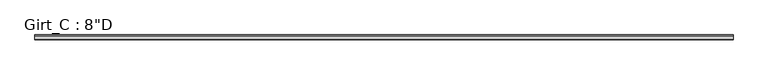
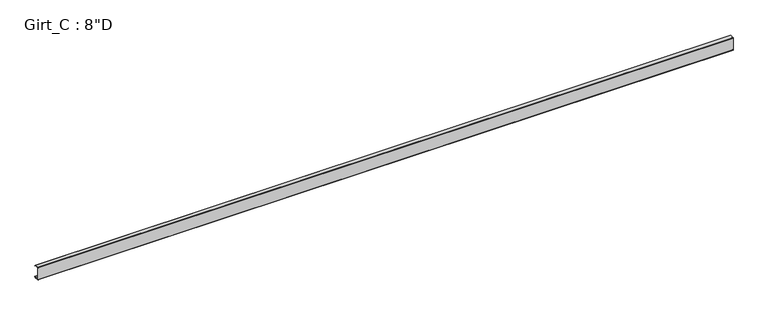
"""IFC4 building model written with IfcOpenShell, lengths in millimetres: beam geometry."""

from ifc_helpers import new_model, si_unit, point, frame, frame_2d, origin, place, context, project, spatial, polyline, circle_curve, trimmed, segment, composite_curve, outline, extrude, source, transform, mapped, element, save


def beam_d1ffb292(model_context):
    return source(origin(), model_context, "Body", "SweptSolid", [
        extrude(outline(composite_curve([segment(polyline([(63.5, 101.6), (75.745104, 87.0068534), (73.6169367, 85.221109), (62.204539, 98.821875), (3.3005807, 98.821875)]), True, "CONTINUOUS"), segment(trimmed(circle_curve(frame_2d((3.3741066, 96.8381931)), 1.9850441), [point((3.3005807, 98.821875))], [point((1.3890625, 96.8381931))], True, "CARTESIAN"), True, "CONTINUOUS"), segment(polyline([(1.3890625, 96.8381931), (1.3890625, -96.8389339)]), True, "CONTINUOUS"), segment(trimmed(circle_curve(frame_2d((3.3748024, -96.8389339)), 1.9857399), [point((1.3890625, -96.8389339))], [point((3.2694106, -98.821875))], True, "CARTESIAN"), True, "CONTINUOUS"), segment(polyline([(3.2694106, -98.821875), (62.204539, -98.821875), (73.6169367, -85.221109), (75.745104, -87.0068534), (63.5, -101.6), (3.3734375, -101.6)]), True, "CONTINUOUS"), segment(trimmed(circle_curve(frame_2d((3.3734375, -96.8375)), 4.7625), [point((3.3734375, -101.6))], [point((-1.3890625, -96.8375))], False, "CARTESIAN"), True, "CONTINUOUS"), segment(polyline([(-1.3890625, -96.8375), (-1.3890625, 96.8375)]), True, "CONTINUOUS"), segment(trimmed(circle_curve(frame_2d((3.3734375, 96.8375)), 4.7625), [point((-1.3890625, 96.8375))], [point((3.3734375, 101.6))], False, "CARTESIAN"), True, "CONTINUOUS"), segment(polyline([(3.3734375, 101.6), (63.5, 101.6)]), True, "CONTINUOUS")], self_intersect=False)), frame((-5383.0884766, 0.0, 0.0), z_axis=(1.0, 0.0, 0.0), x_axis=(0.0, 1.0, 0.0)), (0.0, 0.0, 1.0), 10766.1769531),
    ])


if __name__ == "__main__":
    model = new_model("IFC4")
    model_context = context("Model", 3, world=origin())
    ifc_project = project(units=[si_unit("LENGTHUNIT", "METRE", prefix="MILLI")], contexts=[model_context])
    site = spatial("IfcSite", under=ifc_project)
    building = spatial("IfcBuilding", under=site)
    placement = place(None, origin())
    beam_shape = beam_d1ffb292(model_context)
    element("IfcBeam", 1, ObjectType="Girt_C : 8\"D", at=placement, inside=building, context=model_context, shape_type="MappedRepresentation", body=[
        mapped(beam_shape, transform((0.0, 0.0, 0.0), x_axis=(1.0, 0.0, 0.0), y_axis=(0.0, 1.0, 0.0), z_axis=(0.0, 0.0, 1.0))),
    ])
    save(model, "model.ifc")

# Revit data of these elements
# Type "Girt_C : 8\"D"
#   Web_Thickness = 0' - 0 7/64"
#   Length [instance default] = 10' - 0"
#   Leg_1 = 0' - 2 1/2"
#   Height = 0' - 8"
#   Structural Material [instance default] = none
# Element 1 (IfcBeam, "Girt_C : 8\"D")
#   Structural Material = Steel
#   Materials on its faces: "Steel"
# Materials
#   "Steel": class "Metal", colour RGB 118 118 114, transparency 0, Description = "Steel, mill finish", Cost = 0
